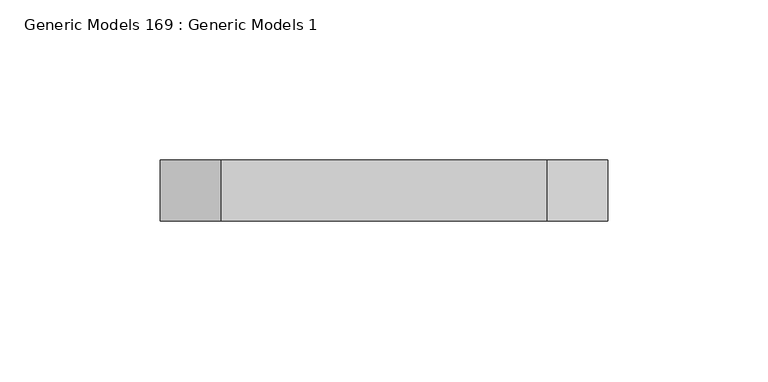
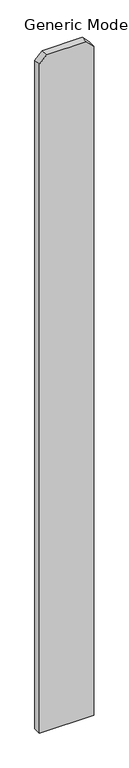
"""IFC4 building model written with IfcOpenShell, lengths in millimetres: proxy geometry, Generic Models 169 : Generic Models 1."""

from ifc_helpers import new_model, si_unit, frame, origin, place, context, project, spatial, polyline, outline, extrude, source, transform, mapped, element, save


def generic_models_169_generic_models_1_1e887b02(model_context):
    return source(origin(), model_context, "Body", "SweptSolid", [
        extrude(outline(polyline([(76.2, -249048.5875), (1885.95, -249048.5875), (1905.0, -249067.6375), (1905.0, -249169.2375), (1885.95, -249188.2875), (76.2, -249188.2875), (76.2, -249048.5875)])), frame((0.0, 547.6875, 0.0), z_axis=(0.0, 1.0, 0.0), x_axis=(0.0, 0.0, 1.0)), (0.0, 0.0, 1.0), 19.05),
    ])


if __name__ == "__main__":
    model = new_model("IFC4")
    model_context = context("Model", 3, world=origin())
    ifc_project = project(units=[si_unit("LENGTHUNIT", "METRE", prefix="MILLI")], contexts=[model_context])
    site = spatial("IfcSite", under=ifc_project)
    building = spatial("IfcBuilding", under=site)
    placement = place(None, origin())
    generic_models_169_generic_models_1_shape = generic_models_169_generic_models_1_1e887b02(model_context)
    element("IfcBuildingElementProxy", 1, Name="Generic Models 169 : Generic Models 1", ObjectType="Generic Models 169 : Generic Models 1", at=placement, inside=building, context=model_context, shape_type="MappedRepresentation", body=[
        mapped(generic_models_169_generic_models_1_shape, transform((0.0, 0.0, 0.0), x_axis=(1.0, 0.0, 0.0), y_axis=(0.0, 1.0, 0.0), z_axis=(0.0, 0.0, 1.0))),
    ])
    save(model, "model.ifc")

# Revit data of these elements
# Element 1 (IfcBuildingElementProxy, "Generic Models 169 : Generic Models 1")
#   Materials on its faces: "VERTICAL 1X6 CEDAR PLANKS W/ CLEAR WOOD SEALER"
# Materials
#   "VERTICAL 1X6 CEDAR PLANKS W/ CLEAR WOOD SEALER": class "Wood", colour RGB 234 198 147, transparency 0, Description = "Pinus Echinata", Cost = 0
